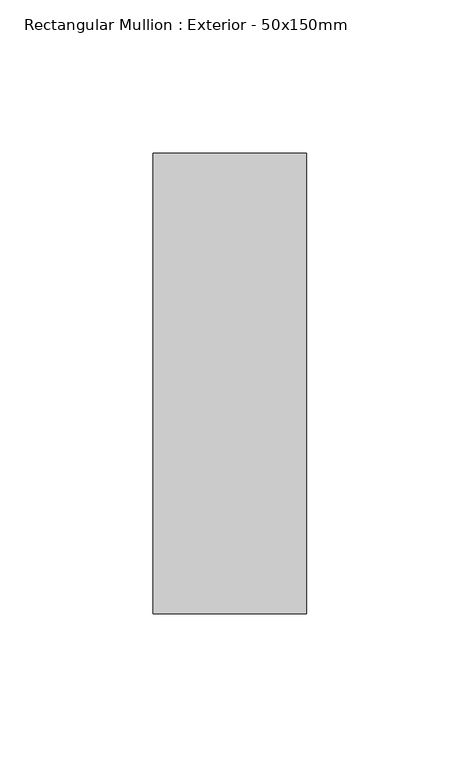
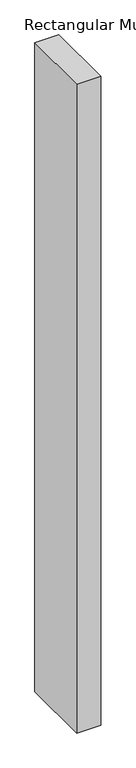
"""IFC4 building model written with IfcOpenShell, lengths in millimetres: member geometry, Rectangular Mullion : Exterior - 50x150mm."""

from ifc_helpers import new_model, si_unit, frame, origin, place, context, project, spatial, polyline, outline, extrude, source, transform, mapped, element, save


def rectangular_mullion_exterior_50x150mm_ae104826(model_context):
    return source(origin(), model_context, "Body", "SweptSolid", [
        extrude(outline(polyline([(25.0, 0.0), (25.0, -150.0), (-25.0, -150.0), (-25.0, 0.0), (25.0, 0.0)])), frame((0.0, 0.0, -1425.0000002), z_axis=(0.0, 0.0, 1.0), x_axis=(1.0, 0.0, 0.0)), (0.0, 0.0, 1.0), 1425.0000002),
    ])


if __name__ == "__main__":
    model = new_model("IFC4")
    model_context = context("Model", 3, world=origin())
    ifc_project = project(units=[si_unit("LENGTHUNIT", "METRE", prefix="MILLI")], contexts=[model_context])
    site = spatial("IfcSite", under=ifc_project)
    building = spatial("IfcBuilding", under=site)
    placement = place(None, origin())
    rectangular_mullion_exterior_50x150mm_shape = rectangular_mullion_exterior_50x150mm_ae104826(model_context)
    element("IfcMember", 1, ObjectType="Rectangular Mullion : Exterior - 50x150mm", at=placement, inside=building, context=model_context, shape_type="MappedRepresentation", body=[
        mapped(rectangular_mullion_exterior_50x150mm_shape, transform((0.0, 0.0, 0.0), x_axis=(1.0, 0.0, 0.0), y_axis=(0.0, 1.0, 0.0), z_axis=(0.0, 0.0, 1.0))),
    ])
    save(model, "model.ifc")

# Revit data of these elements
# Type "Rectangular Mullion : Exterior - 50x150mm"
#   built-in parameter 1007351 = -0.246063 (stored number, unit not read)
#   built-in parameter 1007304 = 0.492126 (stored number, unit not read)
#   built-in parameter 1007301 = 0.082021 (stored number, unit not read)
#   built-in parameter 1007300 = 0.082021 (stored number, unit not read)
# Element 1 (IfcMember, "Rectangular Mullion : Exterior - 50x150mm")
#   Materials on its faces: "Default Frame/Mullion (Interior/Exterior)"
# Materials
#   "Default Frame/Mullion (Interior/Exterior)": class "Generic", colour RGB 205 205 205, transparency 0, Description = "Udefineret karm/ramme materiale", Cost = 0
